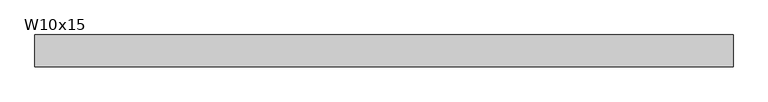
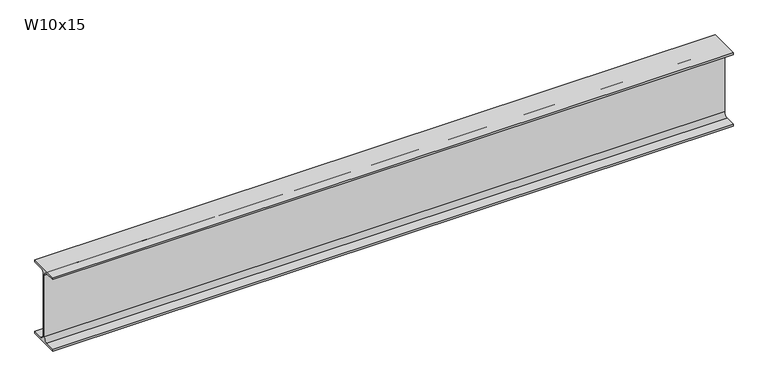
"""IFC4 building model written with IfcOpenShell, lengths in millimetres: beam geometry, RME W-Wide Flange : W10x15."""

from ifc_helpers import new_model, si_unit, point, frame, frame_2d, origin, place, context, project, spatial, polyline, circle_curve, trimmed, segment, composite_curve, outline, extrude, source, transform, mapped, element, save


def w10x15_37cf4fef(model_context):
    return source(origin(), model_context, "Body", "SweptSolid", [
        extrude(outline(composite_curve([segment(polyline([(-50.8, -120.142), (-16.7005, -120.142)]), True, "CONTINUOUS"), segment(trimmed(circle_curve(frame_2d((-16.7005, -106.3625)), 13.7795), [point((-16.7005, -120.142))], [point((-2.921, -106.3625))], True, "CARTESIAN"), True, "CONTINUOUS"), segment(polyline([(-2.921, -106.3625), (-2.921, 106.3625)]), True, "CONTINUOUS"), segment(trimmed(circle_curve(frame_2d((-16.7005, 106.3625)), 13.7795), [point((-2.921, 106.3625))], [point((-16.7005, 120.142))], True, "CARTESIAN"), True, "CONTINUOUS"), segment(polyline([(-16.7005, 120.142), (-50.8, 120.142), (-50.8, 127.0), (50.8, 127.0), (50.8, 120.142), (16.7005, 120.142)]), True, "CONTINUOUS"), segment(trimmed(circle_curve(frame_2d((16.7005, 106.3625)), 13.7795), [point((16.7005, 120.142))], [point((2.921, 106.3625))], True, "CARTESIAN"), True, "CONTINUOUS"), segment(polyline([(2.921, 106.3625), (2.921, -106.3625)]), True, "CONTINUOUS"), segment(trimmed(circle_curve(frame_2d((16.7005, -106.3625)), 13.7795), [point((2.921, -106.3625))], [point((16.7005, -120.142))], True, "CARTESIAN"), True, "CONTINUOUS"), segment(polyline([(16.7005, -120.142), (50.8, -120.142), (50.8, -127.0), (-50.8, -127.0), (-50.8, -120.142)]), True, "CONTINUOUS")], self_intersect=False)), frame((-1079.373, 0.0, 0.0), z_axis=(1.0, 0.0, 0.0), x_axis=(0.0, 1.0, 0.0)), (0.0, 0.0, 1.0), 2222.373),
    ])


if __name__ == "__main__":
    model = new_model("IFC4")
    model_context = context("Model", 3, world=origin())
    ifc_project = project(units=[si_unit("LENGTHUNIT", "METRE", prefix="MILLI")], contexts=[model_context])
    site = spatial("IfcSite", under=ifc_project)
    building = spatial("IfcBuilding", under=site)
    placement = place(None, origin())
    w10x15_shape = w10x15_37cf4fef(model_context)
    element("IfcBeam", 1, ObjectType="RME W-Wide Flange : W10x15", at=placement, inside=building, context=model_context, shape_type="MappedRepresentation", body=[
        mapped(w10x15_shape, transform((0.0, 0.0, 0.0), x_axis=(1.0, 0.0, 0.0), y_axis=(0.0, 1.0, 0.0), z_axis=(0.0, 0.0, 1.0))),
    ])
    save(model, "model.ifc")

# Revit data of these elements
# Type "RME W-Wide Flange : W10x15"
#   WELD P [instance default] = ""
#   WELD LE [instance default] = ""
#   WELD D [instance default] = ""
#   TOP SECTION SIZE [instance default] = ""
#   TOP SECTION LENGTH [instance default] = ""
#   REMARKS [instance default] = ""
#   REINF TYPE [instance default] = ""
#   Nominal Size = "W24"
#   End Bearing Capacity [instance default] = ""
#   BOT SECTION SIZE [instance default] = ""
#   BOT SECTION LENGTH [instance default] = ""
#   Assembly Code = "B10"
#   W = 15
#   Start Extension Calculation [instance default] = 10' - 0"
#   Start Extension [instance default] = -0' - 0 1/2"
#   End Extension Calculation [instance default] = 10' - 0"
#   End Extension [instance default] = -0' - 0 1/2"
#   Length [instance default] = 5' - 0"
#   bf = 0' - 4"
#   d = 0' - 10"
#   k = 0' - 0 13/16"
#   k2 = 0' - 0.5425"
#   tf = 0' - 0.27"
#   tw = 0' - 0.23"
#   A = 0.030625 SF
#   Structural Material [instance default] = Metal - Steel - ASTM A992
# Element 1 (IfcBeam, "RME W-Wide Flange : W10x15")
#   Length = 7' - 6"
#   Materials on its faces: "Metal - Steel - ASTM A992"
# Materials
#   "Metal - Steel - ASTM A992": class "Metal", colour RGB 255 128 0, transparency 0
